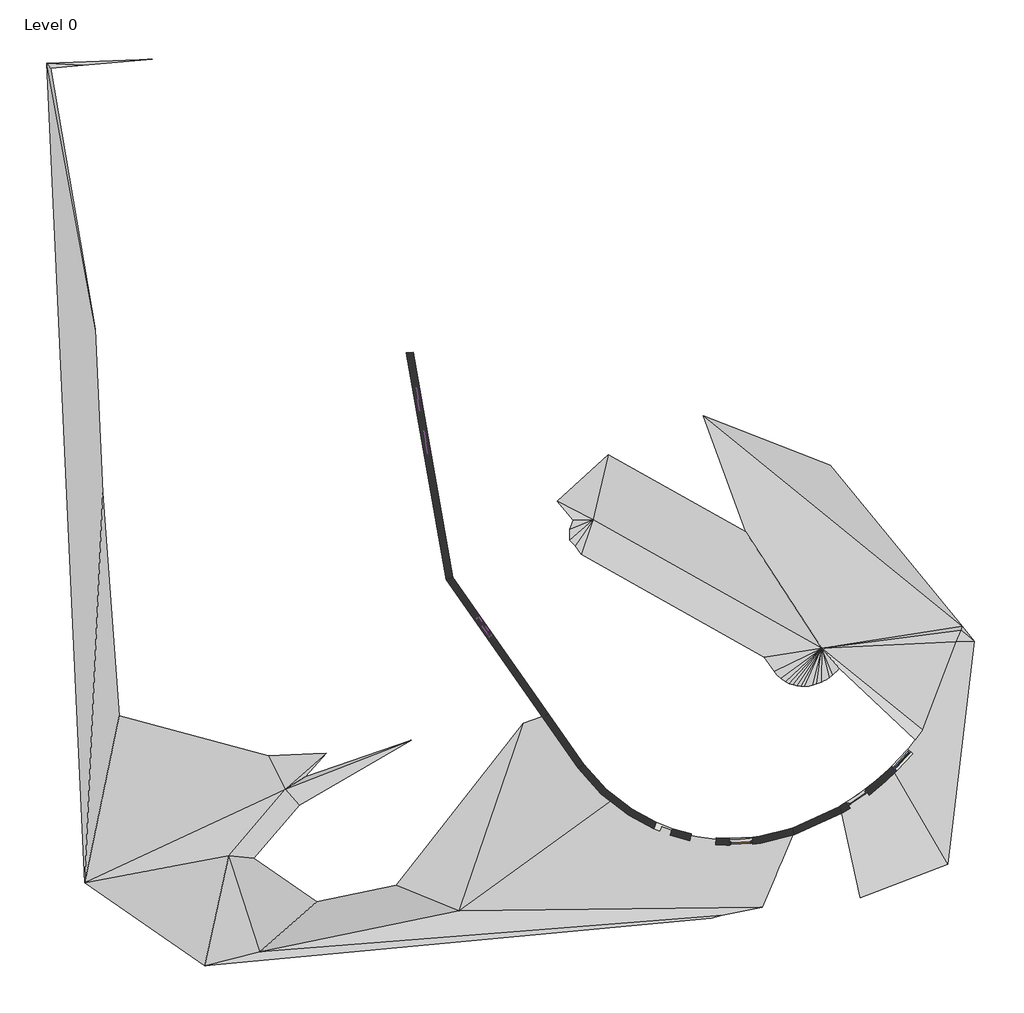
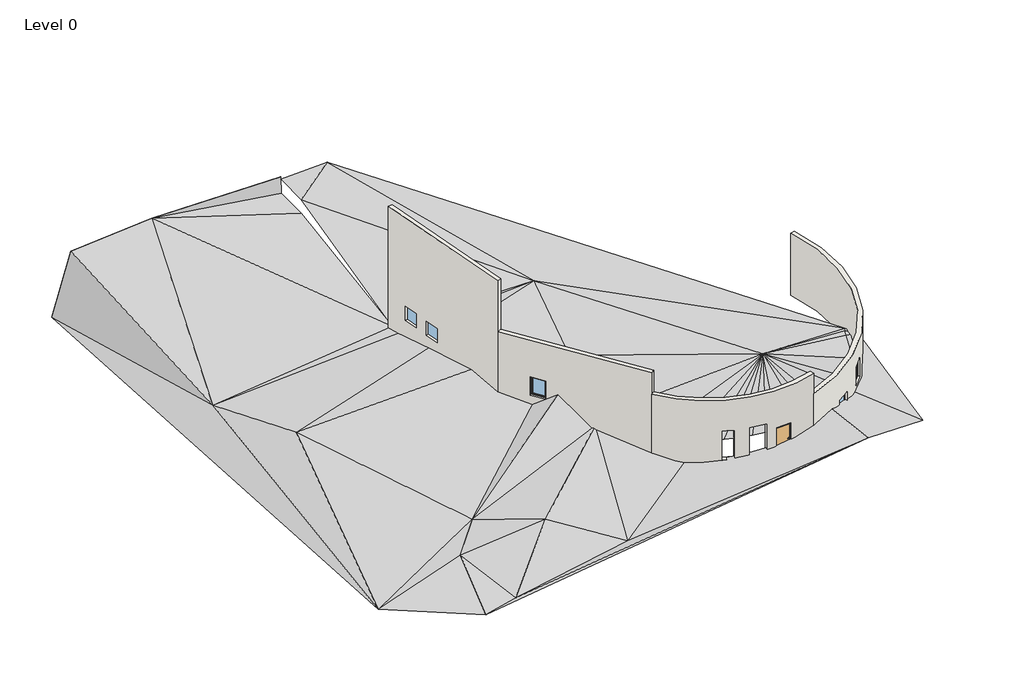
# One storey: 5 windows, 4 walls, 2 proxies, 1 door.
"""IFC4 building model written with IfcOpenShell, lengths in millimetres."""

import ifcopenshell
import ifcopenshell.guid

model = None  # the IFC model being written
_history = None  # IfcOwnerHistory: only IFC2X3 demands one
_inside = {}  # id of a spatial element -> (the spatial element, [elements in it])
_under = {}  # id of a project, library or spatial element -> (it, [spatial elements below it])
_declared = {}  # id of a project -> (the project, [libraries it declares])
_typed = {}  # id of a type object -> (the type object, [elements of that type])
_made_of = {}  # id of a material, layer set ... -> (it, [elements and type objects made of it])


def new_model(schema):
    """Start an empty IFC model of exactly this schema.

    Asked for "IFC4X3", IfcOpenShell would pick the latest addendum, in which some entities
    have other attributes; the version numbers below select the first issue.
    IFC2X3 requires an IfcOwnerHistory on every rooted entity: one is made here for all.
    """
    global model, _history
    if schema == "IFC4X3":
        model = ifcopenshell.file(schema_version=(4, 3, 0, 0))
    else:
        model = ifcopenshell.file(schema=schema)
    _inside.clear()
    _under.clear()
    _declared.clear()
    _typed.clear()
    _made_of.clear()
    _history = None
    if model.schema == "IFC2X3":
        org = make("IfcOrganization", Name="unknown")
        user = make(
            "IfcPersonAndOrganization",
            ThePerson=make("IfcPerson", FamilyName="unknown"),
            TheOrganization=org,
        )
        app = make(
            "IfcApplication",
            ApplicationDeveloper=org,
            Version="unknown",
            ApplicationFullName="unknown",
            ApplicationIdentifier="unknown",
        )
        _history = make(
            "IfcOwnerHistory",
            OwningUser=user,
            OwningApplication=app,
            ChangeAction="ADDED",
            CreationDate=0,
        )
    return model


def make(cls, **values):
    """One entity of the class cls with the attributes given. An attribute that is None is left unset."""
    return model.create_entity(
        cls, **{name: value for name, value in values.items() if value is not None}
    )


def rooted(cls, **values):
    """An entity with a GlobalId (a new one), such as an element, a storey or a relation."""
    return make(cls, GlobalId=ifcopenshell.guid.new(), OwnerHistory=_history, **values)


def si_unit(unit_type, name, prefix=None):
    """IfcSIUnit, for example si_unit("LENGTHUNIT", "METRE", prefix="MILLI")."""
    return make("IfcSIUnit", UnitType=unit_type, Prefix=prefix, Name=name)


def assignment(units):
    """IfcUnitAssignment: the units of a project."""
    return None if units is None else make("IfcUnitAssignment", Units=units)


def point(xyz):
    """IfcCartesianPoint."""
    return None if xyz is None else make("IfcCartesianPoint", Coordinates=xyz)


def direction(xyz):
    """IfcDirection."""
    return None if xyz is None else make("IfcDirection", DirectionRatios=xyz)


def frame(location, z_axis=None, x_axis=None):
    """IfcAxis2Placement3D, a coordinate frame: its origin and axes. An axis left out is left unset."""
    return make(
        "IfcAxis2Placement3D",
        Location=point(location),
        Axis=direction(z_axis),
        RefDirection=direction(x_axis),
    )


def frame_2d(location, x_axis=None):
    """IfcAxis2Placement2D, a coordinate frame in the plane: its origin and x axis."""
    return make(
        "IfcAxis2Placement2D", Location=point(location), RefDirection=direction(x_axis)
    )


def origin():
    """The frame at (0, 0, 0) with its axes left unset."""
    return frame((0.0, 0.0, 0.0))


def origin_with_axes():
    """The frame at (0, 0, 0) with the z axis (0, 0, 1) and the x axis (1, 0, 0) written out."""
    return frame((0.0, 0.0, 0.0), z_axis=(0.0, 0.0, 1.0), x_axis=(1.0, 0.0, 0.0))


def place(relative_to, where):
    """IfcLocalPlacement: puts the frame where relative to a parent placement (None: the world)."""
    return make(
        "IfcLocalPlacement", PlacementRelTo=relative_to, RelativePlacement=where
    )


def context(
    kind, dimensions, precision=None, world=None, true_north=None, identifier=None
):
    """IfcGeometricRepresentationContext, for example the 3D "Model" context."""
    return make(
        "IfcGeometricRepresentationContext",
        ContextIdentifier=identifier,
        ContextType=kind,
        CoordinateSpaceDimension=dimensions,
        Precision=precision,
        WorldCoordinateSystem=world,
        TrueNorth=true_north,
    )


def project(units=None, contexts=None):
    """IfcProject with its units and contexts."""
    return rooted(
        "IfcProject",
        Name="project",
        RepresentationContexts=contexts,
        UnitsInContext=assignment(units),
    )


def spatial(cls, under=None, at=None, **own):
    """A site, building, storey or space (cls), placed at a placement, below another one or the project."""
    s = rooted(cls, ObjectPlacement=at, **own)
    if under is not None:
        _under.setdefault(under.id(), (under, []))[1].append(s)
    return s


def polyline(points):
    """IfcPolyline through the points."""
    return make("IfcPolyline", Points=[point(p) for p in points])


def point_list(points):
    """IfcCartesianPointList2D or 3D."""
    cls = (
        "IfcCartesianPointList2D" if len(points[0]) == 2 else "IfcCartesianPointList3D"
    )
    return make(cls, CoordList=points)


def circle_curve(where, radius):
    """IfcCircle in the frame where."""
    return make("IfcCircle", Position=where, Radius=radius)


def trimmed(basis, trim1, trim2, sense, master):
    """IfcTrimmedCurve: the piece of a basis curve between two trims."""
    return make(
        "IfcTrimmedCurve",
        BasisCurve=basis,
        Trim1=trim1,
        Trim2=trim2,
        SenseAgreement=sense,
        MasterRepresentation=master,
    )


def segment(curve, same_sense, transition):
    """IfcCompositeCurveSegment."""
    return make(
        "IfcCompositeCurveSegment",
        Transition=transition,
        SameSense=same_sense,
        ParentCurve=curve,
    )


def composite_curve(segments, self_intersect=None):
    """IfcCompositeCurve: segments joined end to end."""
    return make("IfcCompositeCurve", Segments=segments, SelfIntersect=self_intersect)


def outline(outer, holes=None, kind="AREA"):
    """IfcArbitraryClosedProfileDef: a profile drawn as a closed curve; with holes, ...WithVoids."""
    if holes is None:
        return make("IfcArbitraryClosedProfileDef", ProfileType=kind, OuterCurve=outer)
    return make(
        "IfcArbitraryProfileDefWithVoids",
        ProfileType=kind,
        OuterCurve=outer,
        InnerCurves=holes,
    )


def extrude(swept, where, along, depth):
    """IfcExtrudedAreaSolid: the profile swept, set in the frame where, extruded along a direction by depth."""
    return make(
        "IfcExtrudedAreaSolid",
        SweptArea=swept,
        Position=where,
        ExtrudedDirection=direction(along),
        Depth=depth,
    )


def faces_of(points, faces, orient=None, outer=None):
    """IfcFace entities. A face is a list of loops; a loop is a list of indices into points, from 0.

    orient and outer hold one flag for each loop. By default every Orientation is true, the
    first loop of a face is its IfcFaceOuterBound and the others are IfcFaceBound.
    """
    made = []
    for i, loops in enumerate(faces):
        bounds = []
        for j, loop in enumerate(loops):
            is_outer = j == 0 if outer is None else outer[i][j]
            bounds.append(
                make(
                    "IfcFaceOuterBound" if is_outer else "IfcFaceBound",
                    Bound=make("IfcPolyLoop", Polygon=[points[k] for k in loop]),
                    Orientation=True if orient is None else orient[i][j],
                )
            )
        made.append(make("IfcFace", Bounds=bounds))
    return made


def faceted_brep(points, faces, orient=None, outer=None, voids=None):
    """IfcFacetedBrep: a solid bounded by flat faces; with voids (closed shells), ...WithVoids."""
    shared = [point(p) for p in points]
    hull = make("IfcClosedShell", CfsFaces=faces_of(shared, faces, orient, outer))
    if voids is None:
        return make("IfcFacetedBrep", Outer=hull)
    return make(
        "IfcFacetedBrepWithVoids",
        Outer=hull,
        Voids=[
            make(cls, CfsFaces=faces_of(shared, fs, o, b)) for cls, fs, o, b in voids
        ],
    )


def triangles(points, corners, closed=None, point_numbers=None):
    """IfcTriangulatedFaceSet: each triangle names its three corners, points numbered from 1."""
    return make(
        "IfcTriangulatedFaceSet",
        Coordinates=point_list(points),
        Closed=closed,
        CoordIndex=corners,
        PnIndex=point_numbers,
    )


def shape(context_of_items, identifier, shape_type, items):
    """IfcShapeRepresentation: the items that make up one representation, for example the "Body"."""
    return make(
        "IfcShapeRepresentation",
        ContextOfItems=context_of_items,
        RepresentationIdentifier=identifier,
        RepresentationType=shape_type,
        Items=items,
    )


def source(mapping_origin, context_of_items, identifier, shape_type, items):
    """IfcRepresentationMap: a shape defined once, which mapped items show again and again."""
    return make(
        "IfcRepresentationMap",
        MappingOrigin=mapping_origin,
        MappedRepresentation=shape(context_of_items, identifier, shape_type, items),
    )


def transform(
    local_origin,
    x_axis=None,
    y_axis=None,
    z_axis=None,
    scale=None,
    scale2=None,
    scale3=None,
    uniform=True,
):
    """IfcCartesianTransformationOperator3D, or its non-uniform kind. x_axis, y_axis, z_axis: its Axis1, 2, 3."""
    if uniform:
        return make(
            "IfcCartesianTransformationOperator3D",
            Axis1=direction(x_axis),
            Axis2=direction(y_axis),
            LocalOrigin=point(local_origin),
            Scale=scale,
            Axis3=direction(z_axis),
        )
    return make(
        "IfcCartesianTransformationOperator3DnonUniform",
        Axis1=direction(x_axis),
        Axis2=direction(y_axis),
        LocalOrigin=point(local_origin),
        Scale=scale,
        Axis3=direction(z_axis),
        Scale2=scale2,
        Scale3=scale3,
    )


def mapped(mapping_source, mapping_target):
    """IfcMappedItem: shows the shape of a source again, moved by a transform."""
    return make(
        "IfcMappedItem", MappingSource=mapping_source, MappingTarget=mapping_target
    )


def made_of(thing, what):
    """Note that an element or type object is made of a material, layer set ...; save() writes the relation."""
    if what is not None:
        _made_of.setdefault(what.id(), (what, []))[1].append(thing)
    return thing


def element(
    cls,
    number,
    at=None,
    inside=None,
    cuts=None,
    type_object=None,
    material=None,
    context=None,
    identifier="Body",
    shape_type=None,
    held_by="IfcProductDefinitionShape",
    body=None,
    shapes=None,
    **own,
):
    """One element of the class cls, such as IfcWall. Its Tag is "e" and its number.

    at: its placement. inside: the storey or other place that contains it. cuts: it is an
    opening in that element (IfcRelVoidsElement). A single representation is given by context,
    identifier, shape_type and body (its items); several are given by shapes. held_by: the class
    of the entity that holds the representations. save() writes the other relations.
    """
    e = rooted(cls, Tag="e%d" % number, ObjectPlacement=at, **own)
    if body is not None:
        shapes = [shape(context, identifier, shape_type, body)]
    if shapes is not None:
        e.Representation = make(held_by, Representations=shapes)
    if inside is not None:
        _inside.setdefault(inside.id(), (inside, []))[1].append(e)
    if cuts is not None:
        rooted(
            "IfcRelVoidsElement", RelatingBuildingElement=cuts, RelatedOpeningElement=e
        )
    if type_object is not None:
        _typed.setdefault(type_object.id(), (type_object, []))[1].append(e)
    return made_of(e, material)


def aggregate(whole, parts):
    """IfcRelAggregates: a whole, such as a stair, and the parts it consists of."""
    return rooted("IfcRelAggregates", RelatingObject=whole, RelatedObjects=parts)


def save(model, path):
    """Write the relations noted so far, then the file.

    IfcRelAggregates (storeys below a building ...), IfcRelContainedInSpatialStructure (elements
    in a storey), IfcRelDefinesByType, IfcRelAssociatesMaterial and IfcRelDeclares: one each for
    every whole, place, type object, material and project.
    """
    for whole, parts in _under.values():
        aggregate(whole, parts)
    for where, things in _inside.values():
        rooted(
            "IfcRelContainedInSpatialStructure",
            RelatedElements=things,
            RelatingStructure=where,
        )
    for kind, things in _typed.values():
        rooted("IfcRelDefinesByType", RelatedObjects=things, RelatingType=kind)
    for what, things in _made_of.values():
        rooted("IfcRelAssociatesMaterial", RelatedObjects=things, RelatingMaterial=what)
    for by, libraries in _declared.values():
        rooted("IfcRelDeclares", RelatingContext=by, RelatedDefinitions=libraries)
    model.write(path)


def plane_surface(at):
    """IfcPlane: the flat surface through the origin of the frame at, square to its z axis."""
    return make("IfcPlane", Position=at)


def cylinder_surface(at, radius):
    """IfcCylindricalSurface: all points at the distance radius from the z axis of the frame at."""
    return make("IfcCylindricalSurface", Position=at, Radius=radius)


def revolved_surface(curve, axis_point, axis_direction):
    """IfcSurfaceOfRevolution: the curve turned about the line through axis_point along axis_direction."""
    return make(
        "IfcSurfaceOfRevolution",
        SweptCurve=make("IfcArbitraryOpenProfileDef", ProfileType="CURVE", Curve=curve),
        AxisPosition=make("IfcAxis1Placement", Location=point(axis_point), Axis=direction(axis_direction)),
    )


def advanced_brep(points, edges, surfaces, faces):
    """IfcAdvancedBrep: a solid bounded by faces that lie on surfaces and meet in shared edges.

    An edge is (start, end): straight between two places in points (the first is 0);
    or (start, end, curve); or (start, end, curve, False) where it runs against its curve.
    A face is (place in surfaces, loops), or (place, loops, False) where it looks against
    its surface's normal. A loop lists edges by number (the first is 1), with a minus sign
    where the edge is run from its end to its start. The first loop is the outer one.
    """
    corners = [point(p) for p in points]
    vertices = [make("IfcVertexPoint", VertexGeometry=c) for c in corners]
    made = []
    for start, end, *more in edges:
        made.append(
            make(
                "IfcEdgeCurve",
                EdgeStart=vertices[start],
                EdgeEnd=vertices[end],
                EdgeGeometry=more[0] if more else make("IfcPolyline", Points=[corners[start], corners[end]]),
                SameSense=more[1] if len(more) > 1 else True,
            )
        )
    hull = []
    for where, loops, *sense in faces:
        bounds = []
        for j, loop in enumerate(loops):
            ring = [make("IfcOrientedEdge", EdgeElement=made[abs(k) - 1], Orientation=k > 0) for k in loop]
            bounds.append(
                make(
                    "IfcFaceOuterBound" if j == 0 else "IfcFaceBound",
                    Bound=make("IfcEdgeLoop", EdgeList=ring),
                    Orientation=True,
                )
            )
        hull.append(make("IfcAdvancedFace", Bounds=bounds, FaceSurface=surfaces[where], SameSense=sense[0] if sense else True))
    return make("IfcAdvancedBrep", Outer=make("IfcClosedShell", CfsFaces=hull))


def single_door_d10_bed63a48(model_context):
    return source(origin(), model_context, "Body", "SolidModel", [
        advanced_brep(
        [(-400.0, -5.0, 1057.5), (-390.0, -5.0, 1067.5), (-400.0, -5.0, 1077.5), (-280.0, -5.0, 1077.5), (-280.0, -5.0, 1057.5), (-400.0, -15.0, 1077.5), (-410.0, -15.0, 1067.5), (-400.0, -15.0, 1057.5), (-280.0, -15.0, 1057.5), (-280.0, -15.0, 1077.5), (-390.0, 45.0, 1067.5), (-410.0, 45.0, 1067.5)],
        [
            (0, 1, circle_curve(frame((-400.0, -5.0, 1067.5), z_axis=(0.0, -1.0, 0.0), x_axis=(0.0, 0.0, 1.0)), 10.0)),
            (1, 2, circle_curve(frame((-400.0, -5.0, 1067.5), z_axis=(0.0, -1.0, 0.0), x_axis=(0.0, 0.0, 1.0)), 10.0)),
            (2, 3),
            (3, 4),
            (4, 0),
            (5, 6, circle_curve(frame((-400.0, -15.0, 1067.5), z_axis=(0.0, -1.0, 0.0), x_axis=(0.0, 0.0, 1.0)), 10.0)),
            (6, 7, circle_curve(frame((-400.0, -15.0, 1067.5), z_axis=(0.0, -1.0, 0.0), x_axis=(0.0, 0.0, 1.0)), 10.0)),
            (7, 8),
            (8, 9),
            (9, 5),
            (4, 8),
            (7, 0),
            (3, 9),
            (2, 5),
            (10, 11, circle_curve(frame((-400.0, 45.0, 1067.5), z_axis=(0.0, 1.0, 0.0), x_axis=(0.0, 0.0, 1.0)), 10.0)),
            (11, 10, circle_curve(frame((-400.0, 45.0, 1067.5), z_axis=(0.0, 1.0, 0.0), x_axis=(0.0, 0.0, 1.0)), 10.0)),
            (11, 6),
            (1, 10),
        ],
        [
            plane_surface(frame((-400.0, -5.0, 1057.5), z_axis=(0.0, 1.0, 0.0), x_axis=(1.0, 0.0, 0.0))),
            plane_surface(frame((-400.0, -15.0, 1057.5), z_axis=(0.0, -1.0, 0.0), x_axis=(-1.0, 0.0, 0.0))),
            plane_surface(frame((-400.0, -5.0, 1057.5), z_axis=(0.0, 0.0, -1.0), x_axis=(0.0, -1.0, 0.0))),
            plane_surface(frame((-280.0, -5.0, 1057.5), z_axis=(1.0, 0.0, 0.0), x_axis=(0.0, -1.0, 0.0))),
            plane_surface(frame((-280.0, -5.0, 1077.5), z_axis=(0.0, 0.0, 1.0), x_axis=(0.0, -1.0, 0.0))),
            plane_surface(frame((-400.0, 45.0, 1077.5), z_axis=(0.0, 1.0, 0.0), x_axis=(-1.0, 0.0, 0.0))),
            cylinder_surface(frame((-400.0, -15.0, 1067.5), z_axis=(0.0, 1.0, 0.0), x_axis=(0.0, 0.0, 1.0)), 10.0),
        ],
        [
            (0, [[1, 2, 3, 4, 5]]),
            (1, [[6, 7, 8, 9, 10]]),
            (2, [[11, -8, 12, -5]]),
            (3, [[13, -9, -11, -4]]),
            (4, [[14, -10, -13, -3]]),
            (5, [[15, 16]]),
            (6, [[17, -6, -14, -2, 18, -16]]),
            (6, [[-18, -1, -12, -7, -17, -15]]),
        ],
    ),
        advanced_brep(
        [(-400.0, 165.0, 1057.5), (-410.0, 165.0, 1067.5), (-400.0, 165.0, 1077.5), (-280.0, 165.0, 1077.5), (-280.0, 165.0, 1057.5), (-400.0, 155.0, 1077.5), (-390.0, 155.0, 1067.5), (-400.0, 155.0, 1057.5), (-280.0, 155.0, 1057.5), (-280.0, 155.0, 1077.5), (-410.0, 105.0, 1067.5), (-390.0, 105.0, 1067.5)],
        [
            (0, 1, circle_curve(frame((-400.0, 165.0, 1067.5), z_axis=(0.0, 1.0, 0.0), x_axis=(1.0, 0.0, 0.0)), 10.0)),
            (1, 2, circle_curve(frame((-400.0, 165.0, 1067.5), z_axis=(0.0, 1.0, 0.0), x_axis=(1.0, 0.0, 0.0)), 10.0)),
            (2, 3),
            (3, 4),
            (4, 0),
            (5, 6, circle_curve(frame((-400.0, 155.0, 1067.5), z_axis=(0.0, 1.0, 0.0), x_axis=(1.0, 0.0, 0.0)), 10.0)),
            (6, 7, circle_curve(frame((-400.0, 155.0, 1067.5), z_axis=(0.0, 1.0, 0.0), x_axis=(1.0, 0.0, 0.0)), 10.0)),
            (7, 8),
            (8, 9),
            (9, 5),
            (4, 8),
            (7, 0),
            (3, 9),
            (2, 5),
            (10, 11, circle_curve(frame((-400.0, 105.0, 1067.5), z_axis=(0.0, -1.0, 0.0), x_axis=(1.0, 0.0, 0.0)), 10.0)),
            (11, 10, circle_curve(frame((-400.0, 105.0, 1067.5), z_axis=(0.0, -1.0, 0.0), x_axis=(1.0, 0.0, 0.0)), 10.0)),
            (10, 1),
            (6, 11),
        ],
        [
            plane_surface(frame((-400.0, 165.0, 1057.5), z_axis=(0.0, 1.0, 0.0), x_axis=(1.0, 0.0, 0.0))),
            plane_surface(frame((-400.0, 155.0, 1057.5), z_axis=(0.0, -1.0, 0.0), x_axis=(-1.0, 0.0, 0.0))),
            plane_surface(frame((-400.0, 165.0, 1057.5), z_axis=(0.0, 0.0, -1.0), x_axis=(0.0, -1.0, 0.0))),
            plane_surface(frame((-280.0, 165.0, 1057.5), z_axis=(1.0, 0.0, 0.0), x_axis=(0.0, -1.0, 0.0))),
            plane_surface(frame((-280.0, 165.0, 1077.5), z_axis=(0.0, 0.0, 1.0), x_axis=(0.0, -1.0, 0.0))),
            plane_surface(frame((-390.0, 105.0, 1067.5), z_axis=(0.0, -1.0, 0.0), x_axis=(0.0, 0.0, -1.0))),
            cylinder_surface(frame((-400.0, 105.0, 1067.5), z_axis=(0.0, 1.0, 0.0), x_axis=(1.0, 0.0, 0.0)), 10.0),
        ],
        [
            (0, [[1, 2, 3, 4, 5]]),
            (1, [[6, 7, 8, 9, 10]]),
            (2, [[11, -8, 12, -5]]),
            (3, [[13, -9, -11, -4]]),
            (4, [[14, -10, -13, -3]]),
            (5, [[15, 16]]),
            (6, [[17, -1, -12, -7, 18, -15]]),
            (6, [[-18, -6, -14, -2, -17, -16]]),
        ],
    ),
        extrude(outline(composite_curve([segment(trimmed(circle_curve(frame_2d((1067.5, -400.0)), 20.0), [point((1047.5, -400.0))], [point((1087.5, -400.0))], False, "CARTESIAN"), True, "CONTINUOUS"), segment(trimmed(circle_curve(frame_2d((1067.5, -400.0)), 20.0), [point((1087.5, -400.0))], [point((1047.5, -400.0))], False, "CARTESIAN"), True, "CONTINUOUS")], self_intersect=False)), frame((0.0, 45.0, 0.0), z_axis=(0.0, 1.0, 0.0), x_axis=(0.0, 0.0, 1.0)), (0.0, 0.0, 1.0), 5.0),
        extrude(outline(composite_curve([segment(trimmed(circle_curve(frame_2d((992.5, -400.0)), 20.0), [point((972.5, -400.0))], [point((1012.5, -400.0))], False, "CARTESIAN"), True, "CONTINUOUS"), segment(trimmed(circle_curve(frame_2d((992.5, -400.0)), 20.0), [point((1012.5, -400.0))], [point((972.5, -400.0))], False, "CARTESIAN"), True, "CONTINUOUS")], self_intersect=False)), frame((0.0, 45.0, 0.0), z_axis=(0.0, 1.0, 0.0), x_axis=(0.0, 0.0, 1.0)), (0.0, 0.0, 1.0), 5.0),
        extrude(outline(composite_curve([segment(trimmed(circle_curve(frame_2d((1067.5, -400.0)), 20.0), [point((1047.5, -400.0))], [point((1087.5, -400.0))], False, "CARTESIAN"), True, "CONTINUOUS"), segment(trimmed(circle_curve(frame_2d((1067.5, -400.0)), 20.0), [point((1087.5, -400.0))], [point((1047.5, -400.0))], False, "CARTESIAN"), True, "CONTINUOUS")], self_intersect=False)), frame((0.0, 100.0, 0.0), z_axis=(0.0, 1.0, 0.0), x_axis=(0.0, 0.0, 1.0)), (0.0, 0.0, 1.0), 5.0),
        extrude(outline(composite_curve([segment(trimmed(circle_curve(frame_2d((992.5, -400.0)), 20.0), [point((972.5, -400.0))], [point((1012.5, -400.0))], False, "CARTESIAN"), True, "CONTINUOUS"), segment(trimmed(circle_curve(frame_2d((992.5, -400.0)), 20.0), [point((1012.5, -400.0))], [point((972.5, -400.0))], False, "CARTESIAN"), True, "CONTINUOUS")], self_intersect=False)), frame((0.0, 100.0, 0.0), z_axis=(0.0, 1.0, 0.0), x_axis=(0.0, 0.0, 1.0)), (0.0, 0.0, 1.0), 5.0),
        extrude(outline(polyline([(445.0, 50.0), (-445.0, 50.0), (-445.0, 100.0), (445.0, 100.0), (445.0, 50.0)])), frame((0.0, 0.0, 10.0), z_axis=(0.0, 0.0, 1.0), x_axis=(1.0, 0.0, 0.0)), (0.0, 0.0, 1.0), 2030.0),
        extrude(outline(polyline([(2110.0, 505.0), (2110.0, -505.0), (0.0, -505.0), (0.0, -445.0), (2040.0, -445.0), (2040.0, 445.0), (0.0, 445.0), (0.0, 505.0), (2110.0, 505.0)])), frame((0.0, 5.0, 0.0), z_axis=(0.0, 1.0, 0.0), x_axis=(0.0, 0.0, 1.0)), (0.0, 0.0, 1.0), 95.0),
        extrude(outline(polyline([(-445.0, 5.0), (-445.0, 100.0), (445.0, 100.0), (445.0, 5.0), (-445.0, 5.0)])), origin_with_axes(), (0.0, 0.0, 1.0), 10.0),
    ])


def window_10x10_03730955(model_context):
    return source(origin(), model_context, "Body", "SweptSolid", [
        extrude(outline(polyline([(575.0, 2.0), (-435.0, 2.0), (-435.0, 18.0), (575.0, 18.0), (575.0, 2.0)])), frame((0.0, 0.0, 800.0), z_axis=(0.0, 0.0, 1.0), x_axis=(1.0, 0.0, 0.0)), (0.0, 0.0, 1.0), 1010.0),
    ])


def single_window_e1c0cfdf(model_context):
    return source(origin(), model_context, "Body", "SweptSolid", [
        extrude(outline(polyline([(510.0, -6.75), (-370.0, -6.75), (-370.0, 9.25), (510.0, 9.25), (510.0, -6.75)])), frame((0.0, 0.0, 865.0), z_axis=(0.0, 0.0, 1.0), x_axis=(1.0, 0.0, 0.0)), (0.0, 0.0, 1.0), 1180.0),
        extrude(outline(polyline([(2045.0, 510.0), (2045.0, -370.0), (865.0, -370.0), (865.0, 510.0), (2045.0, 510.0)]), holes=[polyline([(915.0, 460.0), (915.0, -320.0), (1995.0, -320.0), (1995.0, 460.0), (915.0, 460.0)])]), frame((0.0, -25.0, 0.0), z_axis=(0.0, 1.0, 0.0), x_axis=(0.0, 0.0, 1.0)), (0.0, 0.0, 1.0), 52.5),
        extrude(outline(polyline([(800.0, -435.0), (800.0, 575.0), (2110.0, 575.0), (2110.0, -435.0), (800.0, -435.0)]), holes=[polyline([(865.0, 510.0), (865.0, -370.0), (2045.0, -370.0), (2045.0, 510.0), (865.0, 510.0)])]), frame((0.0, -25.0, 0.0), z_axis=(0.0, 1.0, 0.0), x_axis=(0.0, 0.0, 1.0)), (0.0, 0.0, 1.0), 105.0),
    ])


model = new_model("IFC4")

# Units and contexts
model_context = context("Model", 3, world=origin())
ifc_project = project(units=[si_unit("LENGTHUNIT", "METRE", prefix="MILLI")], contexts=[model_context])

# Site, building, storey
site = spatial("IfcSite", under=ifc_project)
building = spatial("IfcBuilding", under=site)
storey = spatial("IfcBuildingStorey", under=building, Name="Level 0", Elevation=0.0)

# Proxies
placement = place(None, origin())
element("IfcBuildingElementProxy", 1, Name="Building Element Proxy", at=placement, inside=storey, context=model_context, shape_type="Tessellation", body=[
    triangles([(1194.2396049, 50000.4270996, 0.0), (2856.2117065, 14298.8016357, 0.0), (8088.3464127, 10667.0849396, 0.0), (35693.2166748, 13277.7686096, 1500.0000114), (40466.0276733, 15099.0109314, 0.0), (41635.5655884, 24824.626593, 0.0), (41110.0488281, 25465.9083801, 123.7306289), (41049.8525024, 25309.1016724, 58.7363403), (40849.92052, 24788.2543945, 118.1794325), (39380.4288208, 20960.0950378, 270.8285089), (38767.289502, 20161.0368347, 349.0404319), (38086.8403381, 19418.4577423, 438.4613182), (37999.8014648, 19338.7009827, 450.1764462), (37344.2624084, 18738.0085785, 678.1842585), (36545.2042053, 18124.8704224, 948.64275), (35695.7467529, 17583.7069427, 1229.2203186), (35431.5419495, 17446.169989, 1314.5578423), (34802.3594238, 17118.6388184, 1269.8306305), (33871.8348267, 16733.2030426, 1199.8463848), (32911.2609009, 16430.3354828, 1123.9192606), (32075.0956604, 16255.3740692, 1054.3887663), (31224.6917542, 16174.1697235, 979.9247795), (30370.5252869, 16187.7235474, 901.4449041), (29523.1235229, 16295.8681091, 819.9162323), (28692.9323364, 16497.270932, 736.3434992), (27890.1766846, 16789.4496094, 651.7565838), (27124.7536377, 17168.804361, 567.197828), (26406.0928528, 17630.6598907, 483.7092467), (25966.4220154, 17987.8532043, 429.7389582), (25743.0519287, 18169.3235229, 472.6455688), (25143.8001343, 18778.1596161, 608.0284753), (24615.7230652, 19449.6639771, 749.764773), (22428.3077454, 22573.615155, 1393.7781521), (21126.1174622, 24433.3365234, 3200.0000244), (20137.9591736, 25844.5736389, 1954.736935), (18899.0324707, 27613.9447083, 2195.907098), (18498.3546021, 29886.301355, 2500.0000191), (17796.520697, 33866.6002625, 1929.4147888), (17329.2306152, 36516.7315247, 1500.0000114), (17170.6042511, 37416.3487061, 1402.2508907), (17170.6042511, 48195.5837769, 3000.0000229), (17170.6042511, 50462.0128784, 3000.0000229), (17170.6042511, 50582.3497192, 3000.0000229), (17170.6042511, 50614.9012207, 4159.4257645), (19168.1613922, 13067.7116638, 0.0), (10488.9737183, 11282.6299255, 0.0), (14613.1266357, 14914.3466217, 2000.0000153), (1994.4484646, 49138.6657471, 5000.0000381), (7842.128302, 49692.655188, 5000.0000381), (9134.773819, 15468.3372253, 1000.0000076), (11596.9549255, 18361.4001709, 1000.0000076), (5995.4927628, 29441.2145691, 2500.0000191), (3841.0841492, 35535.1123718, 1500.0000114)], [[50, 2, 3], [45, 46, 4], [50, 3, 46], [50, 47, 51], [47, 50, 46], [51, 47, 33], [50, 51, 2], [46, 45, 47], [52, 2, 51], [45, 31, 32], [31, 45, 30], [45, 32, 33], [36, 51, 35], [34, 51, 33], [51, 34, 35], [45, 33, 47], [46, 3, 4], [52, 51, 36], [49, 48, 53], [53, 48, 1], [52, 53, 2], [53, 40, 49], [1, 49, 44], [49, 1, 48], [43, 44, 49], [53, 52, 39], [53, 1, 2], [38, 39, 52], [37, 38, 52], [42, 43, 49], [40, 41, 49], [42, 49, 41], [39, 40, 53], [52, 36, 37], [23, 24, 4], [22, 23, 4], [26, 27, 45], [26, 45, 25], [25, 45, 24], [20, 21, 4], [4, 21, 22], [16, 17, 4], [19, 20, 4], [17, 18, 4], [19, 4, 18], [4, 5, 16], [4, 24, 45], [28, 29, 45], [14, 5, 13], [15, 5, 14], [16, 5, 15], [29, 30, 45], [11, 12, 5], [10, 11, 5], [8, 9, 6], [6, 7, 8], [9, 10, 6], [10, 5, 6], [5, 12, 13], [27, 28, 45]], closed=False),
])
element("IfcBuildingElementProxy", 2, Name="Building Element Proxy", at=placement, inside=storey, context=model_context, shape_type="Tessellation", body=[
    triangles([(20399.2525269, 50739.0796875, 4000.0000305), (17170.6042511, 50614.9012207, 4000.0000305), (17170.6042511, 50582.3497192, 4000.0000305), (17170.6042511, 50462.0128784, 4000.0000305), (17170.6042511, 48195.5837769, 4000.0000305), (17170.6042511, 37416.3487061, 1402.2508907), (17329.2306152, 36516.7315247, 1500.0000114), (17796.520697, 33866.6002625, 1929.4147888), (18498.3546021, 29886.301355, 2500.0000191), (18899.0324707, 27613.9447083, 2195.907098), (20137.9591736, 25844.5736389, 1954.736935), (21126.1174622, 24433.3365234, 2000.0000153), (22428.3077454, 22573.615155, 2000.0000153), (24615.7230652, 19449.6639771, 2000.0000153), (25143.8001343, 18778.1596161, 2000.0000153), (25743.0519287, 18169.3235229, 2000.0000153), (25966.4220154, 17987.8532043, 2000.0000153), (26406.0928528, 17630.6598907, 2000.0000153), (27124.7536377, 17168.804361, 2000.0000153), (27890.1766846, 16789.4496094, 2000.0000153), (28692.9323364, 16497.270932, 2000.0000153), (29523.1235229, 16295.8681091, 2000.0000153), (30370.5252869, 16187.7235474, 2000.0000153), (31224.6917542, 16174.1697235, 2000.0000153), (32075.0956604, 16255.3740692, 2000.0000153), (32911.2609009, 16430.3354828, 2000.0000153), (33871.8348267, 16733.2030426, 2000.0000153), (34802.3594238, 17118.6388184, 2000.0000153), (35431.5419495, 17446.169989, 2000.0000153), (35695.7467529, 17583.7069427, 2000.0000153), (36545.2042053, 18124.8704224, 2000.0000153), (37344.2624084, 18738.0085785, 2000.0000153), (37999.8014648, 19338.7009827, 2000.0000153), (38086.8403381, 19418.4577423, 2000.0000153), (38767.289502, 20161.0368347, 2000.0000153), (39380.4288208, 20960.0950378, 270.8285089), (40849.92052, 24788.2543945, 118.1794325), (41049.8525024, 25309.1016724, 58.7363403), (41110.0488281, 25465.9083801, 123.7306289), (19783.7063782, 50677.5253052, 4000.0000305), (34987.6736938, 24516.852356, 1000.0000076), (25015.8405029, 30118.3151001, 1000.0000076), (26677.8134766, 37197.0853455, 1500.0000114)], [[42, 11, 12], [42, 9, 10], [11, 42, 10], [42, 12, 13], [41, 13, 14], [15, 16, 17], [14, 15, 41], [13, 41, 42], [17, 41, 15], [5, 40, 4], [40, 3, 4], [2, 3, 40], [5, 6, 43], [43, 7, 8], [42, 8, 9], [43, 8, 42], [1, 40, 5], [5, 43, 1], [1, 43, 39], [40, 1, 2], [43, 42, 41], [6, 7, 43], [41, 17, 18], [41, 21, 22], [21, 41, 20], [41, 19, 20], [22, 23, 41], [41, 24, 25], [25, 26, 41], [41, 27, 28], [27, 41, 26], [41, 23, 24], [41, 28, 29], [30, 31, 41], [41, 32, 33], [32, 41, 31], [41, 33, 34], [30, 41, 29], [35, 36, 41], [41, 36, 37], [39, 41, 38], [38, 41, 37], [34, 35, 41], [41, 39, 43], [19, 41, 18]], closed=False),
])

# Door
single_door_d10_shape = single_door_d10_bed63a48(model_context)
element("IfcDoor", 3, ObjectType="Single Door : D10", at=placement, inside=storey, context=model_context, shape_type="MappedRepresentation", body=[
    mapped(single_door_d10_shape, transform((31467.3212643, 16102.9106723, 150.0), x_axis=(-0.998765862325778, -0.04966640970157782, 0.0), y_axis=(0.04966640970157782, -0.998765862325778, 0.0), z_axis=(0.0, 0.0, 1.0))),
])

# Walls
element("IfcWall", 4, ObjectType="_Skissvägg 300 mm kartong", at=placement, inside=storey, context=model_context, shape_type="Brep", body=[
    faceted_brep([(16870.6039936, 37390.1020904, 692.4489604), (18615.1391385, 27496.3516398, 692.4489604), (18615.1391385, 27496.3516398, 10176.1959387), (16870.6039936, 37390.1020904, 10176.1959387), (17144.5193145, 35836.6511112, 2798.3226773), (17144.5193145, 35836.6511112, 3808.3226773), (17319.9039739, 34841.9952807, 3808.3226773), (17319.9039739, 34841.9952807, 2798.3226773), (17476.1873338, 33955.6683029, 2755.4752166), (17476.1873338, 33955.6683029, 3765.4752166), (17651.5719933, 32961.0124724, 3765.4752166), (17651.5719933, 32961.0124724, 2755.4752166), (17170.6039936, 37416.3486895, 692.4489604), (17170.6039936, 37416.3486895, 10176.1959387), (18899.0324021, 27613.9440799, 10176.1959387), (18899.0324021, 27613.9440799, 692.4489604), (17439.9616404, 35888.7455645, 2798.3226773), (17615.3462998, 34894.089734, 2798.3226773), (17615.3462998, 34894.089734, 3808.3226773), (17439.9616404, 35888.7455645, 3808.3226773), (17771.6296597, 34007.7627562, 2755.4752166), (17947.0143192, 33013.1069257, 2755.4752166), (17947.0143192, 33013.1069257, 3765.4752166), (17771.6296597, 34007.7627562, 3765.4752166)], [[[0, 1, 2, 3], [4, 5, 6, 7], [8, 9, 10, 11]], [[12, 13, 14, 15], [16, 17, 18, 19], [20, 21, 22, 23]], [[1, 0, 12, 15]], [[3, 2, 14, 13]], [[0, 3, 13, 12]], [[2, 1, 15, 14]], [[5, 4, 16, 19]], [[6, 5, 19, 18]], [[7, 6, 18, 17]], [[4, 7, 17, 16]], [[9, 8, 20, 23]], [[10, 9, 23, 22]], [[11, 10, 22, 21]], [[8, 11, 21, 20]]]),
])
element("IfcWall", 5, ObjectType="_Skissvägg 300 mm kartong", at=placement, inside=storey, context=model_context, shape_type="Brep", body=[
    faceted_brep([(18615.1391385, 27496.3516398, 0.0), (24371.3513471, 19275.6286477, 0.0), (24371.3513471, 19275.6286477, 6510.3112693), (18615.1391385, 27496.3516398, 6510.3112693), (19832.9877156, 25757.0836218, 2566.0793778), (19832.9877156, 25757.0836218, 3876.0793778), (20412.2999164, 24929.7400571, 3876.0793778), (20412.2999164, 24929.7400571, 2566.0793778), (18899.0324021, 27613.9440799, 0.0), (18899.0324021, 27613.9440799, 6510.3112693), (24614.336301, 19451.6442087, 6510.3112693), (24614.336301, 19451.6442087, 0.0), (20078.7333289, 25929.1565527, 2566.0793778), (20658.0455296, 25101.812988, 2566.0793778), (20658.0455296, 25101.812988, 3876.0793778), (20078.7333289, 25929.1565527, 3876.0793778)], [[[0, 1, 2, 3], [4, 5, 6, 7]], [[8, 9, 10, 11], [12, 13, 14, 15]], [[1, 0, 8, 11]], [[3, 2, 10, 9]], [[0, 3, 9, 8]], [[5, 4, 12, 15]], [[6, 5, 15, 14]], [[7, 6, 14, 13]], [[4, 7, 13, 12]], [[2, 1, 11, 10]]]),
])
element("IfcWall", 6, ObjectType="_Skissvägg 300 mm kartong", at=placement, inside=storey, context=model_context, shape_type="AdvancedBrep", body=[
    advanced_brep(
    [(40837.7055113, 31345.7050644, 3482.2911487), (33686.684882, 16667.5920095, 3482.2911487), (33784.4798222, 16383.979334, 3482.2911487), (41121.3181868, 31443.5000045, 3482.2911487), (33686.684882, 16667.5920095, -964.9718706), (40837.7055113, 31345.7050644, -964.9718706), (41121.3181868, 31443.5000045, -964.9718706), (33784.4798222, 16383.979334, -964.9718706), (33686.684882, 16667.5920095, 0.0), (38038.4486147, 19370.3506502, 2110.0), (38038.4486147, 19370.3506502, 800.0), (38725.0936409, 20111.0385792, 800.0), (38725.0936409, 20111.0385792, 2110.0), (36044.8513808, 17793.559211, 1431.4367871), (36044.8513808, 17793.559211, 121.4367871), (36876.9340456, 18366.0436553, 121.4367871), (36876.9340456, 18366.0436553, 1431.4367871), (33784.4798222, 16383.979334, 0.0), (38258.6603541, 19166.2062466, 800.0), (38258.6603541, 19166.2062466, 2110.0), (38945.3053802, 19906.8941756, 2110.0), (38945.3053802, 19906.8941756, 800.0), (36215.0550392, 17546.1751728, 121.4367871), (36215.0550392, 17546.1751728, 1431.4367871), (37047.137704, 18118.6596171, 1431.4367871), (37047.137704, 18118.6596171, 121.4367871)],
    [
        (0, 1, circle_curve(frame((29923.1386692, 27582.1588516, 3482.2911487), z_axis=(0.0, 0.0, -1.0), x_axis=(1.0, 0.0, 0.0)), 11545.2176007)),
        (1, 2),
        (2, 3, circle_curve(frame((29923.1386692, 27582.1588516, 3482.2911487), z_axis=(0.0, 0.0, 1.0), x_axis=(1.0, 0.0, 0.0)), 11845.2176007)),
        (3, 0),
        (4, 5, circle_curve(frame((29923.1386692, 27582.1588516, -964.9718706), z_axis=(0.0, 0.0, 1.0), x_axis=(1.0, 0.0, 0.0)), 11545.2176007)),
        (5, 6),
        (6, 7, circle_curve(frame((29923.1386692, 27582.1588516, -964.9718706), z_axis=(0.0, 0.0, -1.0), x_axis=(1.0, 0.0, 0.0)), 11845.2176007)),
        (7, 4),
        (0, 5),
        (4, 8),
        (8, 1),
        (9, 10),
        (10, 11, circle_curve(frame((29923.1386692, 27582.1588516, 800.0), z_axis=(0.0, 0.0, 1.0), x_axis=(1.0, 0.0, 0.0)), 11545.2176007)),
        (11, 12),
        (12, 9, circle_curve(frame((29923.1386692, 27582.1588516, 2110.0), z_axis=(0.0, 0.0, -1.0), x_axis=(1.0, 0.0, 0.0)), 11545.2176007)),
        (13, 14),
        (14, 15, circle_curve(frame((29923.1386692, 27582.1588516, 121.4367871), z_axis=(0.0, 0.0, 1.0), x_axis=(1.0, 0.0, 0.0)), 11545.2176007)),
        (15, 16),
        (16, 13, circle_curve(frame((29923.1386692, 27582.1588516, 1431.4367871), z_axis=(0.0, 0.0, -1.0), x_axis=(1.0, 0.0, 0.0)), 11545.2176007)),
        (7, 17),
        (17, 2),
        (6, 3),
        (18, 19),
        (19, 20, circle_curve(frame((29923.1386692, 27582.1588516, 2110.0), z_axis=(0.0, 0.0, 1.0), x_axis=(1.0, 0.0, 0.0)), 11845.2176007)),
        (20, 21),
        (21, 18, circle_curve(frame((29923.1386692, 27582.1588516, 800.0), z_axis=(0.0, 0.0, -1.0), x_axis=(1.0, 0.0, 0.0)), 11845.2176007)),
        (22, 23),
        (23, 24, circle_curve(frame((29923.1386692, 27582.1588516, 1431.4367871), z_axis=(0.0, 0.0, 1.0), x_axis=(1.0, 0.0, 0.0)), 11845.2176007)),
        (24, 25),
        (25, 22, circle_curve(frame((29923.1386692, 27582.1588516, 121.4367871), z_axis=(0.0, 0.0, -1.0), x_axis=(1.0, 0.0, 0.0)), 11845.2176007)),
        (18, 10),
        (9, 19),
        (12, 20),
        (11, 21),
        (22, 14),
        (13, 23),
        (16, 24),
        (15, 25),
    ],
    [
        plane_surface(frame((41468.3562699, 27582.1588516, 3482.2911487), z_axis=(0.0, 0.0, 1.0), x_axis=(0.0, -1.0, 0.0))),
        plane_surface(frame((41468.3562699, 27582.1588516, -964.9718706), z_axis=(0.0, 0.0, -1.0), x_axis=(0.0, 1.0, 0.0))),
        revolved_surface(polyline([(41468.3562699, 27582.1588516, -964.9718706), (41468.3562699, 27582.1588516, 3482.2911487000006)]), (29923.1386692, 27582.1588516, -964.9718706), (0.0, 0.0, -1.0)),
        plane_surface(frame((33686.684882, 16667.5920095, 3482.2911487), z_axis=(-0.9453755849067383, -0.32598313370823695, 0.0), x_axis=(0.0, 0.0, -1.0))),
        cylinder_surface(frame((29923.1386692, 27582.1588516, -964.9718706), z_axis=(0.0, 0.0, 1.0), x_axis=(1.0, 0.0, 0.0)), 11845.2176007),
        plane_surface(frame((41121.3181868, 31443.5000045, 3482.2911487), z_axis=(-0.3259831337082196, 0.9453755849067443, 0.0), x_axis=(0.0, 0.0, -1.0))),
        plane_surface(frame((38258.6603541, 19166.2062466, 800.0), z_axis=(0.6798465605231474, 0.7333543850996234, 0.0), x_axis=(-0.7333543850996234, 0.6798465605231474, 0.0))),
        plane_surface(frame((38258.6603541, 19166.2062466, 2110.0), z_axis=(0.0, 0.0, -1.0), x_axis=(-0.7333543850992733, 0.679846560523525, 0.0))),
        plane_surface(frame((38945.3053802, 19906.8941756, 2110.0), z_axis=(-0.6798465605231734, -0.7333543850995992, 0.0), x_axis=(-0.7333543850995992, 0.6798465605231734, 0.0))),
        plane_surface(frame((38945.3053802, 19906.8941756, 800.0), z_axis=(0.0, 0.0, 1.0000000000000002), x_axis=(-0.7333543850992584, 0.6798465605235411, 0.0))),
        plane_surface(frame((35351.0682523, 18801.9445394, 121.4367871), z_axis=(0.8238442225385569, 0.5668162815144256, 0.0), x_axis=(0.5668162815144256, -0.8238442225385569, 0.0))),
        plane_surface(frame((35351.0682523, 18801.9445394, 1431.4367871), z_axis=(0.0, 0.0, -1.0), x_axis=(0.5668162815144256, -0.8238442225385569, 0.0))),
        plane_surface(frame((36183.150917, 19374.4289837, 1431.4367871), z_axis=(-0.8238442225385569, -0.5668162815144256, 0.0), x_axis=(0.5668162815144256, -0.8238442225385569, 0.0))),
        plane_surface(frame((36183.150917, 19374.4289837, 121.4367871), z_axis=(0.0, 0.0, 1.0), x_axis=(0.5668162815144256, -0.8238442225385569, 0.0))),
    ],
    [
        (0, [[1, 2, 3, 4]]),
        (1, [[5, 6, 7, 8]]),
        (2, [[-1, 9, -5, 10, 11], [12, 13, 14, 15], [16, 17, 18, 19]]),
        (3, [[-2, -11, -10, -8, 20, 21]]),
        (4, [[-3, -21, -20, -7, 22], [23, 24, 25, 26], [27, 28, 29, 30]]),
        (5, [[-4, -22, -6, -9]]),
        (6, [[-23, 31, -12, 32]]),
        (7, [[-24, -32, -15, 33]]),
        (8, [[-25, -33, -14, 34]]),
        (9, [[-26, -34, -13, -31]]),
        (10, [[35, -16, 36, -27]]),
        (11, [[-36, -19, 37, -28]]),
        (12, [[-37, -18, 38, -29]]),
        (13, [[-35, -30, -38, -17]]),
    ],
),
])
element("IfcWall", 7, ObjectType="_Skissvägg 300 mm kartong", at=placement, inside=storey, context=model_context, shape_type="AdvancedBrep", body=[
    advanced_brep(
    [(33686.684882, 16667.5920095, 4961.1425213), (24614.336301, 19451.6442087, 4961.1425213), (24371.3513471, 19275.6286477, 4961.1425213), (33784.4798222, 16383.979334, 4961.1425213), (33686.684882, 16667.5920095, 0.0), (33784.4798222, 16383.979334, 0.0), (30353.7492537, 15957.4706108, 0.0), (30379.1230562, 16256.3956351, 0.0), (24371.3513471, 19275.6286477, 0.0), (24614.336301, 19451.6442087, 0.0), (29289.7771163, 16424.539019, 0.0), (29223.8376716, 16131.8754073, 0.0), (33686.684882, 16667.5920095, 3482.2911487), (30379.1230562, 16256.3956351, 2763.8282876), (29289.7771163, 16424.539019, 2763.8282876), (28472.5697914, 16654.5143408, 2748.5936941), (27777.2088602, 16926.9450256, 2748.5936941), (27777.2088602, 16926.9450256, 663.8065623), (28472.5697914, 16654.5143408, 663.8065623), (30955.466239, 16228.2131799, 2260.0), (30955.466239, 16228.2131799, 150.0), (31964.21976, 16278.3762537, 150.0), (31964.21976, 16278.3762537, 2260.0), (29223.8376716, 16131.8754073, 2763.8282876), (30353.7492537, 15957.4706108, 2763.8282876), (33784.4798222, 16383.979334, 3482.2911487), (27654.943596, 16652.9902753, 2748.5936941), (28376.1987466, 16370.4146722, 2748.5936941), (28376.1987466, 16370.4146722, 663.8065623), (27654.943596, 16652.9902753, 663.8065623), (30970.3944652, 15928.0142561, 150.0), (30970.3944652, 15928.0142561, 2260.0), (31979.1479862, 15978.1773299, 2260.0), (31979.1479862, 15978.1773299, 150.0)],
    [
        (0, 1, circle_curve(frame((31060.5087616, 24283.7001119, 4961.1425213), z_axis=(0.0, 0.0, -1.0), x_axis=(1.0, 0.0, 0.0)), 8056.1717734)),
        (1, 2),
        (2, 3, circle_curve(frame((31060.5087616, 24283.7001119, 4961.1425213), z_axis=(0.0, 0.0, 1.0), x_axis=(1.0, 0.0, 0.0)), 8356.1717734)),
        (3, 0),
        (4, 5),
        (5, 6, circle_curve(frame((31060.5087616, 24283.7001119, 0.0), z_axis=(0.0, 0.0, -1.0), x_axis=(1.0, 0.0, 0.0)), 8356.1717734)),
        (6, 7),
        (7, 4, circle_curve(frame((31060.5087616, 24283.7001119, 0.0), z_axis=(0.0, 0.0, 1.0), x_axis=(1.0, 0.0, 0.0)), 8056.1717734)),
        (8, 9),
        (9, 10, circle_curve(frame((31060.5087616, 24283.7001119, 0.0), z_axis=(0.0, 0.0, 1.0), x_axis=(1.0, 0.0, 0.0)), 8056.1717734)),
        (10, 11),
        (11, 8, circle_curve(frame((31060.5087616, 24283.7001119, 0.0), z_axis=(0.0, 0.0, -1.0), x_axis=(1.0, 0.0, 0.0)), 8356.1717734)),
        (0, 12),
        (12, 4),
        (7, 13),
        (13, 14, circle_curve(frame((31060.5087616, 24283.7001119, 2763.8282876), z_axis=(0.0, 0.0, -1.0), x_axis=(1.0, 0.0, 0.0)), 8056.1717734)),
        (14, 10),
        (9, 1),
        (15, 16, circle_curve(frame((31060.5087616, 24283.7001119, 2748.5936941), z_axis=(0.0, 0.0, -1.0), x_axis=(1.0, 0.0, 0.0)), 8056.1717734)),
        (16, 17),
        (17, 18, circle_curve(frame((31060.5087616, 24283.7001119, 663.8065623), z_axis=(0.0, 0.0, 1.0), x_axis=(1.0, 0.0, 0.0)), 8056.1717734)),
        (18, 15),
        (19, 20),
        (20, 21, circle_curve(frame((31060.5087616, 24283.7001119, 150.0), z_axis=(0.0, 0.0, 1.0), x_axis=(1.0, 0.0, 0.0)), 8056.1717734)),
        (21, 22),
        (22, 19, circle_curve(frame((31060.5087616, 24283.7001119, 2260.0), z_axis=(0.0, 0.0, -1.0), x_axis=(1.0, 0.0, 0.0)), 8056.1717734)),
        (2, 8),
        (11, 23),
        (23, 24, circle_curve(frame((31060.5087616, 24283.7001119, 2763.8282876), z_axis=(0.0, 0.0, 1.0), x_axis=(1.0, 0.0, 0.0)), 8356.1717734)),
        (24, 6),
        (5, 25),
        (25, 3),
        (26, 27, circle_curve(frame((31060.5087616, 24283.7001119, 2748.5936941), z_axis=(0.0, 0.0, 1.0), x_axis=(1.0, 0.0, 0.0)), 8356.1717734)),
        (27, 28),
        (28, 29, circle_curve(frame((31060.5087616, 24283.7001119, 663.8065623), z_axis=(0.0, 0.0, -1.0), x_axis=(1.0, 0.0, 0.0)), 8356.1717734)),
        (29, 26),
        (30, 31),
        (31, 32, circle_curve(frame((31060.5087616, 24283.7001119, 2260.0), z_axis=(0.0, 0.0, 1.0), x_axis=(1.0, 0.0, 0.0)), 8356.1717734)),
        (32, 33),
        (33, 30, circle_curve(frame((31060.5087616, 24283.7001119, 150.0), z_axis=(0.0, 0.0, -1.0), x_axis=(1.0, 0.0, 0.0)), 8356.1717734)),
        (26, 16),
        (15, 27),
        (28, 18),
        (17, 29),
        (23, 14),
        (13, 24),
        (30, 20),
        (19, 31),
        (22, 32),
        (21, 33),
    ],
    [
        plane_surface(frame((39116.6805351, 24283.7001119, 4961.1425213), z_axis=(0.0, 0.0, 1.0), x_axis=(0.0, -1.0, 0.0))),
        plane_surface(frame((39116.6805351, 24283.7001119, 0.0), z_axis=(0.0, 0.0, -1.0), x_axis=(0.0, 1.0, 0.0))),
        revolved_surface(polyline([(39116.680535, 24283.7001119, 0.0), (39116.680535, 24283.7001119, 4961.1425213)]), (31060.5087616, 24283.7001119, 0.0), (0.0, 0.0, -1.0)),
        cylinder_surface(frame((31060.5087616, 24283.7001119, 0.0), z_axis=(0.0, 0.0, 1.0), x_axis=(1.0, 0.0, 0.0)), 8356.1717734),
        plane_surface(frame((33784.4798222, 16383.979334, 4961.1425213), z_axis=(0.9453755849067228, 0.32598313370828236, 0.0), x_axis=(0.0, 0.0, -1.0))),
        plane_surface(frame((24614.336301, 19451.6442087, 0.0), z_axis=(-0.5866430421458739, 0.8098456279451254, 0.0), x_axis=(-0.8098456279451254, -0.5866430421458739, 0.0))),
        plane_surface(frame((39116.6805351, 24283.7001119, 2748.5936941), z_axis=(0.0, 0.0, -1.0), x_axis=(0.0, -1.0, 0.0))),
        plane_surface(frame((39116.6805351, 24283.7001119, 663.8065623), z_axis=(0.0, 0.0, 1.0), x_axis=(0.0, 1.0, 0.0))),
        plane_surface(frame((27777.2088602, 16926.9450256, 2748.5936941), z_axis=(0.9131825007234545, -0.40755088071608686, 0.0), x_axis=(0.0, 0.0, -1.0))),
        plane_surface(frame((28376.1987466, 16370.4146722, 2748.5936941), z_axis=(-0.9469988954585573, 0.321236816072306, 0.0), x_axis=(0.0, 0.0, -1.0))),
        plane_surface(frame((39116.6805351, 24283.7001119, 2763.8282876), z_axis=(0.0, 0.0, -1.0), x_axis=(0.0, -1.0, 0.0))),
        plane_surface(frame((29289.7771163, 16424.539019, 2763.8282876), z_axis=(0.9755453724014429, -0.21979814918722637, 0.0), x_axis=(0.0, 0.0, -1.0))),
        plane_surface(frame((30353.7492537, 15957.4706108, 2763.8282876), z_axis=(-0.9964167476276317, 0.0845793417281821, 0.0), x_axis=(0.0, 0.0, -1.0))),
        plane_surface(frame((30879.802934, 17749.763189, 150.0), z_axis=(0.9987658623257781, 0.049666409701578124, 0.0), x_axis=(0.049666409701578124, -0.9987658623257781, 0.0))),
        plane_surface(frame((30879.802934, 17749.763189, 2260.0), z_axis=(0.0, 0.0, -1.0000000000000002), x_axis=(0.049666409701578124, -0.9987658623257781, 0.0))),
        plane_surface(frame((31888.5564549, 17799.9262628, 2260.0), z_axis=(-0.9987658623257781, -0.049666409701578124, 0.0), x_axis=(0.049666409701578124, -0.9987658623257781, 0.0))),
        plane_surface(frame((31888.5564549, 17799.9262628, 150.0), z_axis=(0.0, 0.0, 1.0000000000000002), x_axis=(0.049666409701578124, -0.9987658623257781, 0.0))),
    ],
    [
        (0, [[1, 2, 3, 4]]),
        (1, [[5, 6, 7, 8]]),
        (1, [[9, 10, 11, 12]]),
        (2, [[-1, 13, 14, -8, 15, 16, 17, -10, 18], [19, 20, 21, 22], [23, 24, 25, 26]]),
        (3, [[-3, 27, -12, 28, 29, 30, -6, 31, 32], [33, 34, 35, 36], [37, 38, 39, 40]]),
        (4, [[-4, -32, -31, -5, -14, -13]]),
        (5, [[-2, -18, -9, -27]]),
        (6, [[41, -19, 42, -33]]),
        (7, [[43, -21, 44, -35]]),
        (8, [[-41, -36, -44, -20]]),
        (9, [[-42, -22, -43, -34]]),
        (10, [[45, -16, 46, -29]]),
        (11, [[-45, -28, -11, -17]]),
        (12, [[-46, -15, -7, -30]]),
        (13, [[47, -23, 48, -37]]),
        (14, [[-48, -26, 49, -38]]),
        (15, [[-49, -25, 50, -39]]),
        (16, [[-47, -40, -50, -24]]),
    ],
),
])

# Windows
window_10x10_shape = window_10x10_03730955(model_context)
element("IfcWindow", 8, ObjectType="Window_skiss : 10x10", at=placement, inside=storey, context=model_context, shape_type="MappedRepresentation", body=[
    mapped(window_10x10_shape, transform((17367.7774347, 35434.3069653, 1998.3226773), x_axis=(0.1736481776669285, -0.9848077530122084, 0.0), y_axis=(0.9848077530122084, 0.1736481776669285, 0.0), z_axis=(0.0, 0.0, 1.0))),
])
element("IfcWindow", 9, ObjectType="Window_skiss : 10x10", at=placement, inside=storey, context=model_context, shape_type="MappedRepresentation", body=[
    mapped(window_10x10_shape, transform((17699.4454541, 33553.324157, 1955.4752166), x_axis=(0.1736481776669285, -0.9848077530122084, 0.0), y_axis=(0.9848077530122084, 0.1736481776669285, 0.0), z_axis=(0.0, 0.0, 1.0))),
])
single_window_shape = single_window_e1c0cfdf(model_context)
element("IfcWindow", 10, ObjectType="Single Window : 10x13 Inåtgående", at=placement, inside=storey, context=model_context, shape_type="MappedRepresentation", body=[
    mapped(single_window_shape, transform((20205.3662721, 25486.788948, 1766.0793778), x_axis=(0.5735764363510445, -0.8191520442889929, 0.0), y_axis=(0.8191520442889929, 0.5735764363510445, 0.0), z_axis=(0.0, 0.0, 1.0))),
])
element("IfcWindow", 11, ObjectType="Single Window : 10x13 Inåtgående", at=placement, inside=storey, context=model_context, shape_type="MappedRepresentation", body=[
    mapped(single_window_shape, transform((36488.2460599, 17916.5476601, -678.5632129), x_axis=(0.8238442225385567, 0.566816281514426, 0.0), y_axis=(-0.566816281514426, 0.8238442225385567, 0.0), z_axis=(0.0, 0.0, 1.0))),
])
element("IfcWindow", 12, ObjectType="Single Window : 10x13 Inåtgående", at=placement, inside=storey, context=model_context, shape_type="MappedRepresentation", body=[
    mapped(single_window_shape, transform((38444.1850263, 19587.3828237, 0.0), x_axis=(0.6798465605231702, 0.7333543850996022, 0.0), y_axis=(-0.7333543850996022, 0.6798465605231702, 0.0), z_axis=(0.0, 0.0, 1.0))),
])

save(model, "model.ifc")

# Revit data of these elements
# Project information
#   Project Issue Date = "Issue Date"
#   Project Status = "Project Status"
#   Client Name = "Owner"
#   Project Address = "Enter address here"
#   Project Name = "Project Name"
#   Project Number = "Project Number"
# Type "Single Door : D10"
#   Type Mark = "D10"
#   Fire Rating = "EI 120"
#   CQSwingCount = ""
#   CQTypeCount = ""
#   URL = "http://www.cad-q.com"
#   Keynote = "43.CC"
#   Construction Type = "Generell innerdörr"
#   CQOriginalSwingDirection = "Left"
#   Wall Width [instance default] = 200 mm
#   Thickness = 50 mm
#   Inset1000 [instance default] = 1000 mm
#   Inset [instance default] = 0 mm
#   GapTop [instance default] = 20 mm
#   GapLock [instance default] = 10 mm
#   GapHinge [instance default] = 10 mm
#   Gap = 10 mm
#   Frame Width = 990 mm
#   Frame Thickness = 50 mm
#   Frame Height = 2090 mm
#   Frame Depth [instance default] = 95 mm
#   Plan Swing Angle = 90.00°
#   Standard Frame Depth = 95 mm
#   Rough Width = 1010 mm
#   Rough Height = 2110 mm
#   Threshold Height = 10 mm
#   Height [instance default] = 2110 mm
#   Width [instance default] = 1010 mm
#   Panel Height = 2030 mm
#   Panel Width = 890 mm
#   Clear Opening Width [instance default] = 840 mm
#   Threshold = yes
#   MWidth [instance default] = 10
#   MHeight [instance default] = 21
#   Gap Top [instance default] = yes
#   Gap Lock Side [instance default] = yes
#   Gap Hinge Side [instance default] = yes
#   CQReversedRoomAssociation [instance default] = no
#   Material Threshold = none
#   Material Panel = none
#   Material Frame = none
#   Material Exterior = none
#   Handle = element 307872
#   Material Glass = none
#   Door Panel = element 307881
#   Material Hardware = none
#   Operation = ""
#   Wall Closure = (empty or 0)
#   Function = (empty or 0)
#   Assembly Code = ""
# Type "_Skissvägg 300 mm kartong"
#   Keynote = "42.B"
#   URL = "www.nyrens.se"
#   Description = "SKISS"
#   Type Mark = ""
#   Fire Rating = ""
#   Nyr_Ljudklass = ""
#   Layers, outside or top first: 300 mm "Kartong" (function 4)
# Type "Window_skiss : 10x10"
#   Type Mark = "F15"
#   Keynote = "42.D"
#   Construction Type = "Generellt fönster"
#   Analytic Construction = "<None>"
#   Wall Width [instance default] = 350 mm
#   Rough Width = 1010 mm
#   Rough Height = 1010 mm
#   Inset [instance default] = 70 mm
#   Height [instance default] = 1010 mm
#   Width [instance default] = 1010 mm
#   Default Sill Height = 800 mm
#   Material Glass = Plexiglas
#   URL = ""
#   Wall Closure = (empty or 0)
#   Assembly Code = ""
# Type "Single Window : 10x13 Inåtgående"
#   Type Mark = "F2"
#   CQSwingCount = ""
#   URL = "www.cad-q.se"
#   Keynote = "42.D"
#   Construction Type = "Generellt fönster"
#   CQOriginalSwingDirection = "Left"
#   Analytic Construction = "<None>"
#   Wall Width [instance default] = 350 mm
#   Rough Width = 1010 mm
#   Rough Height = 1310 mm
#   Inset1000 [instance default] = 1070 mm
#   Inset [instance default] = 70 mm
#   Height [instance default] = 1310 mm
#   GapTop [instance default] = 15 mm
#   GapSecondary [instance default] = 15 mm
#   GapPrimary [instance default] = 15 mm
#   GapBottom [instance default] = 15 mm
#   Gap = 15 mm
#   Frame Width = 980 mm
#   Frame Thickness = 50 mm
#   Frame Height = 1280 mm
#   Frame Depth = 105 mm
#   Width [instance default] = 1010 mm
#   Default Sill Height = 800 mm
#   Panel Height = 1180 mm
#   Panel Width = 880 mm
#   MWidth [instance default] = 10
#   MHeight [instance default] = 13
#   Gap Top [instance default] = yes
#   Gap Secondary Side [instance default] = yes
#   Gap Primary Side [instance default] = yes
#   Gap Bottom [instance default] = yes
#   Material Interior = Default Window Interior
#   Material Glass = none
#   Material Exterior = none
#   Panel Operation = element 308022
#   Wall Closure = (empty or 0)
#   Assembly Code = ""
# Elements 1, 2 (IfcBuildingElementProxy)
#   Material = none
#   Phase Created = New Construction
# Element 3 (IfcDoor, "Single Door : D10")
#   Width = 1010 mm
#   Inset1000 = 1050 mm
#   Inset = 50 mm
#   Height = 2110 mm
#   GapTop = 20 mm
#   GapLock = 10 mm
#   GapHinge = 10 mm
#   Clear Opening Width = 840 mm
#   MWidth = 10
#   MHeight = 21
#   Gap Top = yes
#   Gap Lock Side = yes
#   Gap Hinge Side = yes
#   CQReversedRoomAssociation = no
#   Phase Created = New Construction
#   Materials on its faces: "Default Hardware", "Door - Frame/Mullion"
# Element 4 (IfcWall, "_Skissvägg 300 mm kartong")
#   built-in parameter 1001111 = 692.449 mm
#   Top Offset = 0 mm
#   Base Offset = 692.449 mm
#   Unconnected Height = 9483.747 mm
#   wall height = 9483.747 mm
#   Phase Created = New Construction
#   Base Constraint = Level 0
#   Materials on its faces: "Kartong"
# Element 5 (IfcWall, "_Skissvägg 300 mm kartong")
#   Top Offset = 0 mm
#   Base Offset = 0 mm
#   Unconnected Height = 6510.311 mm
#   wall height = 6510.311 mm
#   Phase Created = New Construction
#   Base Constraint = Level 0
#   Materials on its faces: "Kartong"
# Element 6 (IfcWall, "_Skissvägg 300 mm kartong")
#   built-in parameter 1001111 = -964.972 mm
#   Top Offset = 0 mm
#   Base Offset = -964.972 mm
#   Unconnected Height = 4447.263 mm
#   wall height = 4447.263 mm
#   Phase Created = New Construction
#   Materials on its faces: "Kartong"
# Element 7 (IfcWall, "_Skissvägg 300 mm kartong")
#   Top Offset = 0 mm
#   Base Offset = 0 mm
#   Unconnected Height = 4961.143 mm
#   wall height = 4961.143 mm
#   Phase Created = New Construction
#   Materials on its faces: "Kartong"
# Element 8 (IfcWindow, "Window_skiss : 10x10")
#   Mark = "37"
#   Width = 1010 mm
#   Inset = 70 mm
#   Height = 1010 mm
#   Phase Created = New Construction
#   Materials on its faces: "Plexiglas"
# Element 9 (IfcWindow, "Window_skiss : 10x10")
#   Mark = "38"
#   Width = 1010 mm
#   Inset = 70 mm
#   Height = 1010 mm
#   Phase Created = New Construction
#   Materials on its faces: "Plexiglas"
# Element 10 (IfcWindow, "Single Window : 10x13 Inåtgående")
#   Mark = "39"
#   Width = 1010 mm
#   Inset1000 = 1070 mm
#   Inset = 70 mm
#   Height = 1310 mm
#   GapTop = 15 mm
#   GapSecondary = 15 mm
#   GapPrimary = 15 mm
#   GapBottom = 15 mm
#   MWidth = 10
#   MHeight = 13
#   Gap Top = yes
#   Gap Secondary Side = yes
#   Gap Primary Side = yes
#   Gap Bottom = yes
#   Phase Created = New Construction
#   Materials on its faces: "Partier - Generell", "Glas - Generellt", "Default Window Interior"
# Element 11 (IfcWindow, "Single Window : 10x13 Inåtgående")
#   Mark = "43"
#   Width = 1010 mm
#   Inset1000 = 1070 mm
#   Inset = 70 mm
#   Height = 1310 mm
#   GapTop = 15 mm
#   GapSecondary = 15 mm
#   GapPrimary = 15 mm
#   GapBottom = 15 mm
#   MWidth = 10
#   MHeight = 13
#   Gap Top = yes
#   Gap Secondary Side = yes
#   Gap Primary Side = yes
#   Gap Bottom = yes
#   Phase Created = New Construction
#   Materials on its faces: "Partier - Generell", "Glas - Generellt", "Default Window Interior"
# Element 12 (IfcWindow, "Single Window : 10x13 Inåtgående")
